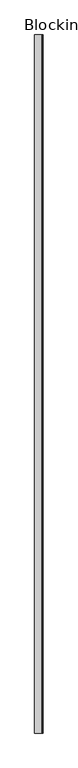
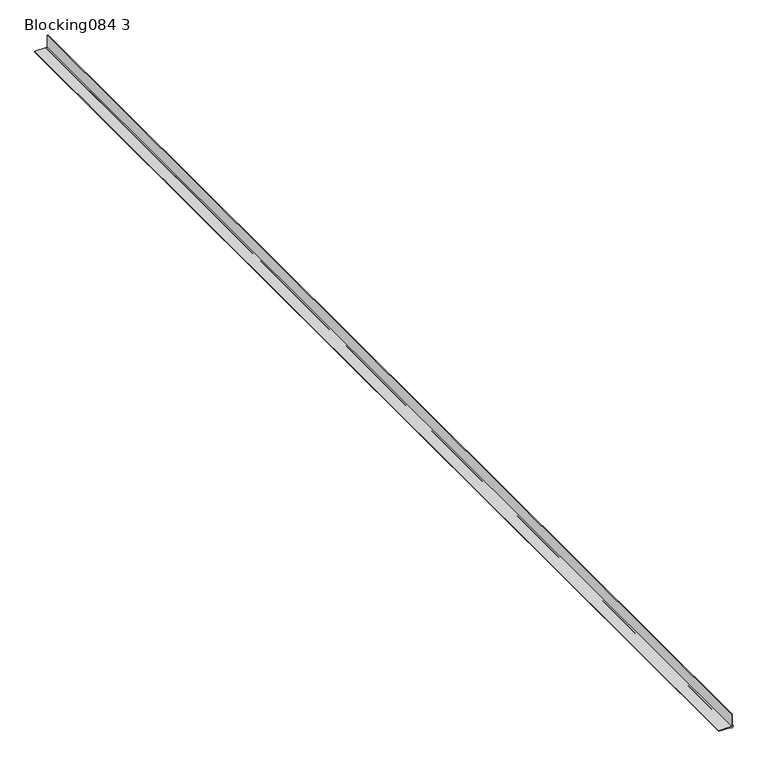
"""IFC4 building model written with IfcOpenShell, lengths in millimetres: proxy geometry, Blocking084 3 : Blocking084 10484."""

from ifc_helpers import new_model, si_unit, point, frame, frame_2d, origin, place, context, project, spatial, polyline, circle_curve, trimmed, segment, composite_curve, outline, extrude, source, transform, mapped, element, save


def blocking084_3_7f017c89(model_context):
    return source(origin(), model_context, "Body", "SweptSolid", [
        extrude(outline(composite_curve([segment(polyline([(42121.2158547, 6211.4587308), (42100.0626708, 6211.4587308), (42100.0626708, 6190.3055469), (42098.7826708, 6190.3055469), (42098.7826708, 6209.1570759)]), True, "CONTINUOUS"), segment(trimmed(circle_curve(frame_2d((42100.0626708, 6211.4587308)), 2.6336316), [point((42098.7826708, 6209.1570759))], [point((42102.3643257, 6212.7387308))], False, "CARTESIAN"), True, "CONTINUOUS"), segment(polyline([(42102.3643257, 6212.7387308), (42121.2158547, 6212.7387308), (42121.2158547, 6211.4587308)]), True, "CONTINUOUS")], self_intersect=False)), frame((0.0, -1052.8912362, 0.0), z_axis=(0.0, 1.0, 0.0), x_axis=(0.0, 0.0, 1.0)), (0.0, 0.0, 1.0), 2000.0),
    ])


if __name__ == "__main__":
    model = new_model("IFC4")
    model_context = context("Model", 3, world=origin())
    ifc_project = project(units=[si_unit("LENGTHUNIT", "METRE", prefix="MILLI")], contexts=[model_context])
    site = spatial("IfcSite", under=ifc_project)
    building = spatial("IfcBuilding", under=site)
    placement = place(None, origin())
    blocking084_3_shape = blocking084_3_7f017c89(model_context)
    element("IfcBuildingElementProxy", 1, Name="Blocking084 3 : Blocking084 10484", ObjectType="Blocking084 3 : Blocking084 10484", at=placement, inside=building, context=model_context, shape_type="MappedRepresentation", body=[
        mapped(blocking084_3_shape, transform((0.0, 0.0, 0.0), x_axis=(1.0, 0.0, 0.0), y_axis=(0.0, 1.0, 0.0), z_axis=(0.0, 0.0, 1.0))),
    ])
    save(model, "model.ifc")

# Revit data of these elements
# Type "Blocking084 3 : Blocking084 10484"
#   NameOverride = "Blocking084"
# Element 1 (IfcBuildingElementProxy, "Blocking084 3 : Blocking084 10484")
#   Materials on its faces: "CORNER BEAD"
# Materials
#   "CORNER BEAD": class "Unassigned", colour RGB 253 236 176, transparency 0, Cost = 0
